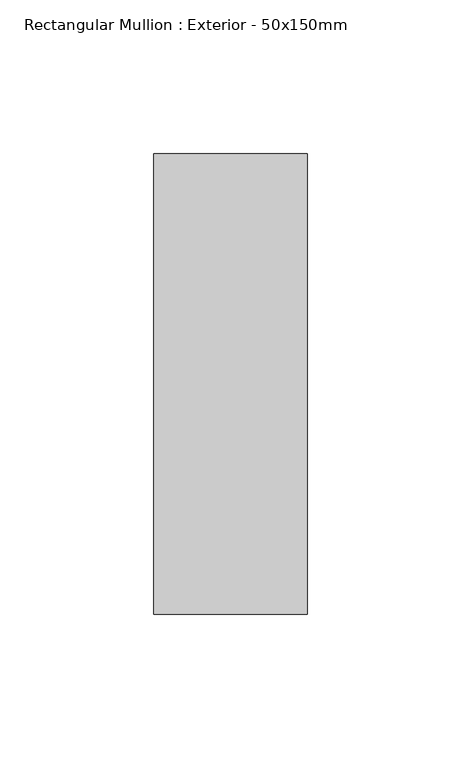
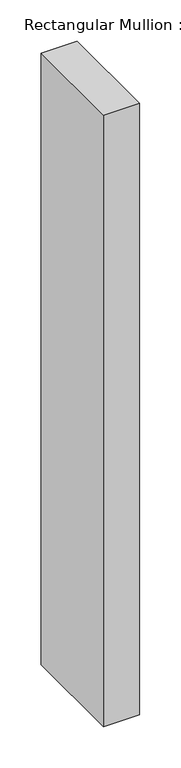
"""IFC4 building model written with IfcOpenShell, lengths in millimetres: member geometry, Rectangular Mullion : Exterior - 50x150mm."""

from ifc_helpers import new_model, si_unit, frame, origin, place, context, project, spatial, polyline, outline, extrude, source, transform, mapped, element, save


def rectangular_mullion_exterior_50x150mm_5b23c5d7(model_context):
    return source(origin(), model_context, "Body", "SweptSolid", [
        extrude(outline(polyline([(0.0, 0.0), (0.0, -150.0), (-50.0, -150.0), (-50.0, 0.0), (0.0, 0.0)])), frame((0.0, 0.0, -900.0), z_axis=(0.0, 0.0, 1.0), x_axis=(1.0, 0.0, 0.0)), (0.0, 0.0, 1.0), 900.0),
    ])


if __name__ == "__main__":
    model = new_model("IFC4")
    model_context = context("Model", 3, world=origin())
    ifc_project = project(units=[si_unit("LENGTHUNIT", "METRE", prefix="MILLI")], contexts=[model_context])
    site = spatial("IfcSite", under=ifc_project)
    building = spatial("IfcBuilding", under=site)
    placement = place(None, origin())
    rectangular_mullion_exterior_50x150mm_shape = rectangular_mullion_exterior_50x150mm_5b23c5d7(model_context)
    element("IfcMember", 1, ObjectType="Rectangular Mullion : Exterior - 50x150mm", at=placement, inside=building, context=model_context, shape_type="MappedRepresentation", body=[
        mapped(rectangular_mullion_exterior_50x150mm_shape, transform((0.0, 0.0, 0.0), x_axis=(1.0, 0.0, 0.0), y_axis=(0.0, 1.0, 0.0), z_axis=(0.0, 0.0, 1.0))),
    ])
    save(model, "model.ifc")

# Revit data of these elements
# Type "Rectangular Mullion : Exterior - 50x150mm"
#   built-in parameter 1007351 = -0.246063 (stored number, unit not read)
#   built-in parameter 1007304 = 0.492126 (stored number, unit not read)
#   built-in parameter 1007301 = 0.082021 (stored number, unit not read)
#   built-in parameter 1007300 = 0.082021 (stored number, unit not read)
# Element 1 (IfcMember, "Rectangular Mullion : Exterior - 50x150mm")
#   Materials on its faces: "Default Frame/Mullion (Interior/Exterior)"
# Materials
#   "Default Frame/Mullion (Interior/Exterior)": class "Generic", colour RGB 205 205 205, transparency 0, Description = "Udefineret karm/ramme materiale", Cost = 0
